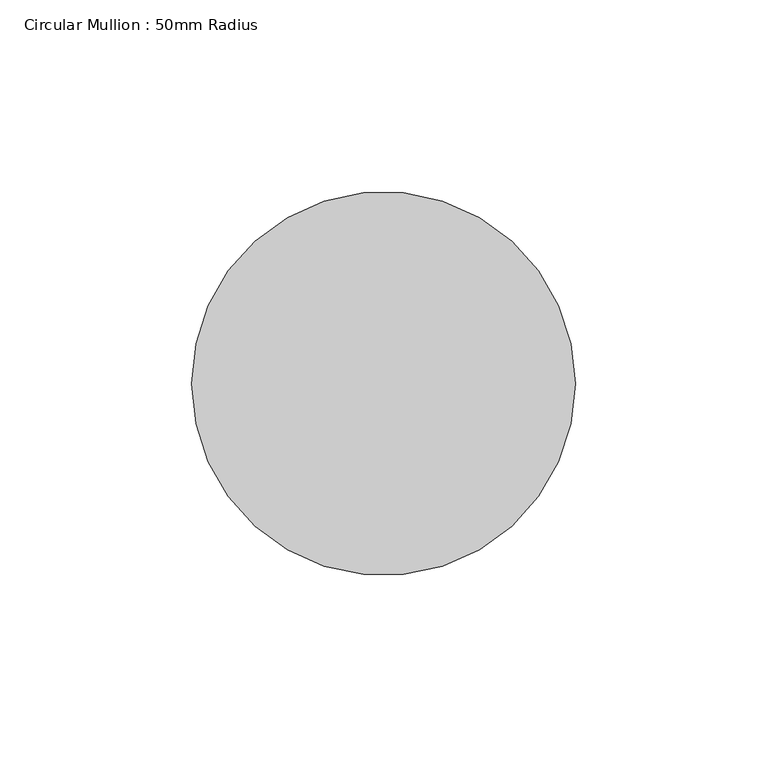
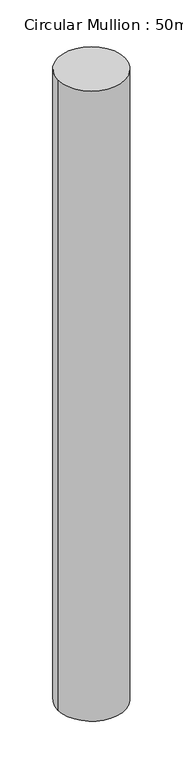
"""IFC4 building model written with IfcOpenShell, lengths in millimetres: member geometry, Circular Mullion : 50mm Radius."""

from ifc_helpers import new_model, si_unit, point, frame, origin, origin_2d, place, context, project, spatial, circle_curve, trimmed, segment, composite_curve, outline, extrude, source, transform, mapped, element, save


def circular_mullion_50mm_radius_7e179ab1(model_context):
    return source(origin(), model_context, "Body", "SweptSolid", [
        extrude(outline(composite_curve([segment(trimmed(circle_curve(origin_2d(), 50.0), [point((50.0, 0.0))], [point((-50.0, 0.0))], False, "CARTESIAN"), True, "CONTINUOUS"), segment(trimmed(circle_curve(origin_2d(), 50.0), [point((-50.0, 0.0))], [point((50.0, 0.0))], False, "CARTESIAN"), True, "CONTINUOUS")], self_intersect=False)), frame((0.0, 0.0, -995.5893904), z_axis=(0.0, 0.0, 1.0), x_axis=(1.0, 0.0, 0.0)), (0.0, 0.0, 1.0), 995.5893904),
    ])


if __name__ == "__main__":
    model = new_model("IFC4")
    model_context = context("Model", 3, world=origin())
    ifc_project = project(units=[si_unit("LENGTHUNIT", "METRE", prefix="MILLI")], contexts=[model_context])
    site = spatial("IfcSite", under=ifc_project)
    building = spatial("IfcBuilding", under=site)
    placement = place(None, origin())
    circular_mullion_50mm_radius_shape = circular_mullion_50mm_radius_7e179ab1(model_context)
    element("IfcMember", 1, ObjectType="Circular Mullion : 50mm Radius", at=placement, inside=building, context=model_context, shape_type="MappedRepresentation", body=[
        mapped(circular_mullion_50mm_radius_shape, transform((0.0, 0.0, 0.0), x_axis=(1.0, 0.0, 0.0), y_axis=(0.0, 1.0, 0.0), z_axis=(0.0, 0.0, 1.0))),
    ])
    save(model, "model.ifc")

# Revit data of these elements
# Type "Circular Mullion : 50mm Radius"
#   built-in parameter 1007350 = 0.164042 (stored number, unit not read)
# Element 1 (IfcMember, "Circular Mullion : 50mm Radius")
#   Materials on its faces: "Aluminium"
# Materials
#   "Aluminium": class "Metal", colour RGB 247 247 247, transparency 0, Description = "Aluminium 6061", Cost = 0
